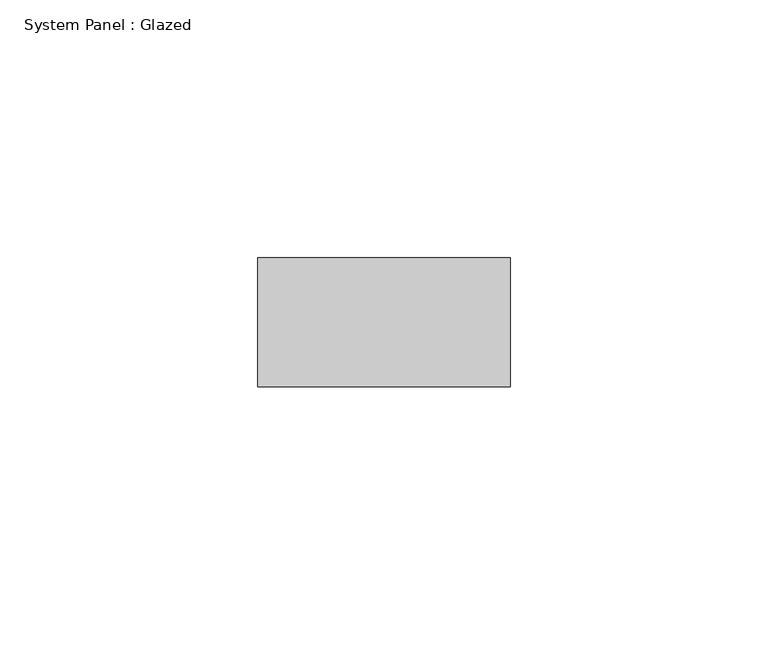
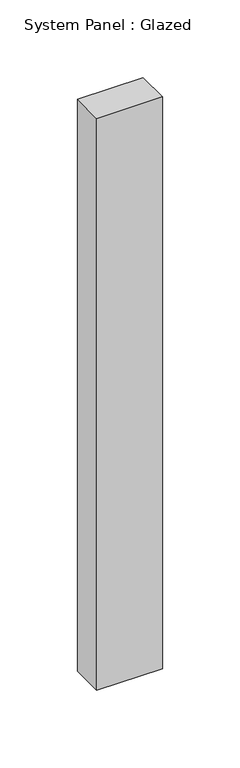
"""IFC4 building model written with IfcOpenShell, lengths in millimetres: plate geometry, System Panel : Glazed."""

from ifc_helpers import new_model, si_unit, origin, origin_with_axes, place, context, project, spatial, polyline, outline, extrude, source, transform, mapped, element, save


def system_panel_glazed_455bb06a(model_context):
    return source(origin(), model_context, "Body", "SweptSolid", [
        extrude(outline(polyline([(24.5092572, -49.5), (-24.5092572, -49.5), (-24.5092572, -24.5), (24.5092572, -24.5), (24.5092572, -49.5)])), origin_with_axes(), (0.0, 0.0, 1.0), 450.0),
    ])


if __name__ == "__main__":
    model = new_model("IFC4")
    model_context = context("Model", 3, world=origin())
    ifc_project = project(units=[si_unit("LENGTHUNIT", "METRE", prefix="MILLI")], contexts=[model_context])
    site = spatial("IfcSite", under=ifc_project)
    building = spatial("IfcBuilding", under=site)
    placement = place(None, origin())
    system_panel_glazed_shape = system_panel_glazed_455bb06a(model_context)
    element("IfcPlate", 1, ObjectType="System Panel : Glazed", at=placement, inside=building, context=model_context, shape_type="MappedRepresentation", body=[
        mapped(system_panel_glazed_shape, transform((0.0, 0.0, 0.0), x_axis=(1.0, 0.0, 0.0), y_axis=(0.0, 1.0, 0.0), z_axis=(0.0, 0.0, 1.0))),
    ])
    save(model, "model.ifc")

# Revit data of these elements
# Type "System Panel : Glazed"
#   Keynote = "H11"
#   Construction Type Id = "GSP4R"
#   Analytic Construction = "1/8 in Pilkington single glazing"
#   Visual Light Transmittance = 0.9
#   Solar Heat Gain Coefficient = 0.86
#   Heat Transfer Coefficient (U) = 6.7069 W/(m²·K)
# Element 1 (IfcPlate, "System Panel : Glazed")
#   Materials on its faces: "Glass"
# Materials
#   "Glass": class "Glass", colour RGB 0 128 192, transparency 0.9, Description = "Soda Lime Glass", Cost = 0
